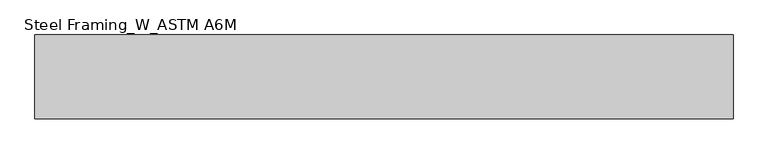
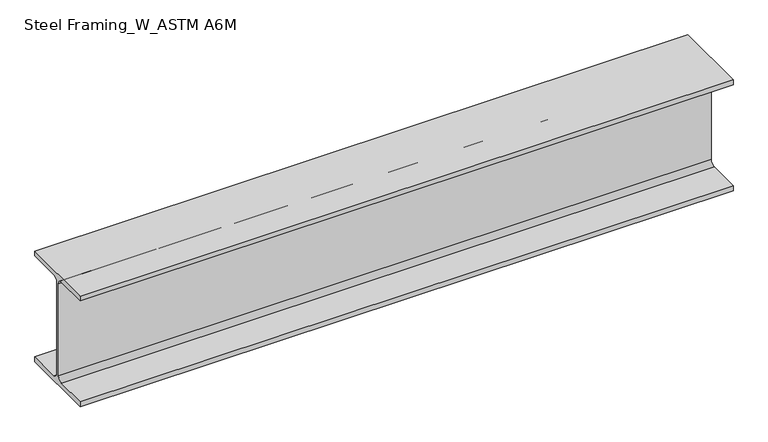
"""IFC4 building model written with IfcOpenShell, lengths in millimetres: beam geometry, Steel Framing_W_ASTM A6M : H_SB_AR_S02_W310x60_B5."""

from ifc_helpers import new_model, si_unit, point, frame, frame_2d, origin, place, context, project, spatial, polyline, circle_curve, trimmed, segment, composite_curve, outline, extrude, source, transform, mapped, element, save


def steel_framing_w_astm_a6m_b2783e68(model_context):
    return source(origin(), model_context, "Body", "SweptSolid", [
        extrude(outline(composite_curve([segment(polyline([(101.5, -137.9), (101.5, -151.0), (-101.5, -151.0), (-101.5, -137.9), (-16.545, -137.9)]), True, "CONTINUOUS"), segment(trimmed(circle_curve(frame_2d((-16.545, -125.1)), 12.8), [point((-16.545, -137.9))], [point((-3.745, -125.1))], True, "CARTESIAN"), True, "CONTINUOUS"), segment(polyline([(-3.745, -125.1), (-3.745, 125.1)]), True, "CONTINUOUS"), segment(trimmed(circle_curve(frame_2d((-16.545, 125.1)), 12.8), [point((-3.745, 125.1))], [point((-16.545, 137.9))], True, "CARTESIAN"), True, "CONTINUOUS"), segment(polyline([(-16.545, 137.9), (-101.5, 137.9), (-101.5, 151.0), (101.5, 151.0), (101.5, 137.9), (16.545, 137.9)]), True, "CONTINUOUS"), segment(trimmed(circle_curve(frame_2d((16.545, 125.1)), 12.8), [point((16.545, 137.9))], [point((3.745, 125.1))], True, "CARTESIAN"), True, "CONTINUOUS"), segment(polyline([(3.745, 125.1), (3.745, -125.1)]), True, "CONTINUOUS"), segment(trimmed(circle_curve(frame_2d((16.545, -125.1)), 12.8), [point((3.745, -125.1))], [point((16.545, -137.9))], True, "CARTESIAN"), True, "CONTINUOUS"), segment(polyline([(16.545, -137.9), (101.5, -137.9)]), True, "CONTINUOUS")], self_intersect=False)), frame((-951.5, 0.0, 0.0), z_axis=(1.0, 0.0, 0.0), x_axis=(0.0, 1.0, 0.0)), (0.0, 0.0, 1.0), 1686.8),
    ])


if __name__ == "__main__":
    model = new_model("IFC4")
    model_context = context("Model", 3, world=origin())
    ifc_project = project(units=[si_unit("LENGTHUNIT", "METRE", prefix="MILLI")], contexts=[model_context])
    site = spatial("IfcSite", under=ifc_project)
    building = spatial("IfcBuilding", under=site)
    placement = place(None, origin())
    steel_framing_w_astm_a6m_shape = steel_framing_w_astm_a6m_b2783e68(model_context)
    element("IfcBeam", 1, ObjectType="Steel Framing_W_ASTM A6M : H_SB_AR_S02_W310x60_B5", at=placement, inside=building, context=model_context, shape_type="MappedRepresentation", body=[
        mapped(steel_framing_w_astm_a6m_shape, transform((0.0, 0.0, 0.0), x_axis=(1.0, 0.0, 0.0), y_axis=(0.0, 1.0, 0.0), z_axis=(0.0, 0.0, 1.0))),
    ])
    save(model, "model.ifc")

# Revit data of these elements
# Type "Steel Framing_W_ASTM A6M : H_SB_AR_S02_W310x60_B5"
#   Type Mark = "B5"
#   Section Name Key = "W12x40"
#   Width = 20.3 cm
#   Web Thickness = 0.749 cm
#   Web Fillet = 1.28 cm
#   Warping Constant = 387000.0 cm⁶
#   Torsional Moment of Inertia = 37.70 cm⁴
#   Section Area = 75.5 cm²
#   Plastic Modulus weak axis = 275.0 cm³
#   Plastic Modulus strong axis = 934.0 cm³
#   Perimeter = 1.38 m²/m
#   Nominal Weight = 60.00 kgf/m
#   Moment of Inertia weak axis = 1840.00 cm⁴
#   Moment of Inertia strong axis = 12800.00 cm⁴
#   Height = 30.2 cm
#   Flange Thickness = 1.31 cm
#   Elastic Modulus weak axis = 180.0 cm³
#   Elastic Modulus strong axis = 844.0 cm³
#   Centroid Vertical = 15.1 cm
#   Centroid Horizontal = 10.15 cm
#   Length [instance default] = 1500 mm
#   Structural Material [instance default] = Steel, 45-345
#   Bolt Spacing = 0
#   Assembly Code = ""
# Element 1 (IfcBeam, "Steel Framing_W_ASTM A6M : H_SB_AR_S02_W310x60_B5")
#   Materials on its faces: "Steel, 45-345"
# Materials
#   "Steel, 45-345": class "Metal", colour RGB 189 187 185, transparency 0, Description = "Steel 345 MPa", Cost = 0
